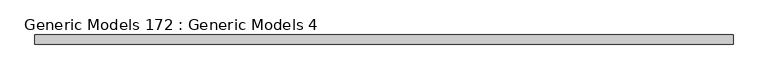
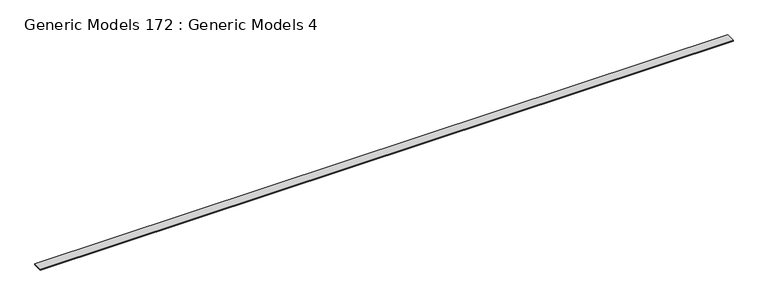
"""IFC4 building model written with IfcOpenShell, lengths in millimetres: proxy geometry, Generic Models 172 : Generic Models 4."""

import ifcopenshell
import ifcopenshell.guid

model = None  # the IFC model being written
_history = None  # IfcOwnerHistory: only IFC2X3 demands one
_inside = {}  # id of a spatial element -> (the spatial element, [elements in it])
_under = {}  # id of a project, library or spatial element -> (it, [spatial elements below it])
_declared = {}  # id of a project -> (the project, [libraries it declares])
_typed = {}  # id of a type object -> (the type object, [elements of that type])
_made_of = {}  # id of a material, layer set ... -> (it, [elements and type objects made of it])


def new_model(schema):
    """Start an empty IFC model of exactly this schema.

    Asked for "IFC4X3", IfcOpenShell would pick the latest addendum, in which some entities
    have other attributes; the version numbers below select the first issue.
    IFC2X3 requires an IfcOwnerHistory on every rooted entity: one is made here for all.
    """
    global model, _history
    if schema == "IFC4X3":
        model = ifcopenshell.file(schema_version=(4, 3, 0, 0))
    else:
        model = ifcopenshell.file(schema=schema)
    _inside.clear()
    _under.clear()
    _declared.clear()
    _typed.clear()
    _made_of.clear()
    _history = None
    if model.schema == "IFC2X3":
        org = make("IfcOrganization", Name="unknown")
        user = make(
            "IfcPersonAndOrganization",
            ThePerson=make("IfcPerson", FamilyName="unknown"),
            TheOrganization=org,
        )
        app = make(
            "IfcApplication",
            ApplicationDeveloper=org,
            Version="unknown",
            ApplicationFullName="unknown",
            ApplicationIdentifier="unknown",
        )
        _history = make(
            "IfcOwnerHistory",
            OwningUser=user,
            OwningApplication=app,
            ChangeAction="ADDED",
            CreationDate=0,
        )
    return model


def make(cls, **values):
    """One entity of the class cls with the attributes given. An attribute that is None is left unset."""
    return model.create_entity(
        cls, **{name: value for name, value in values.items() if value is not None}
    )


def rooted(cls, **values):
    """An entity with a GlobalId (a new one), such as an element, a storey or a relation."""
    return make(cls, GlobalId=ifcopenshell.guid.new(), OwnerHistory=_history, **values)


def si_unit(unit_type, name, prefix=None):
    """IfcSIUnit, for example si_unit("LENGTHUNIT", "METRE", prefix="MILLI")."""
    return make("IfcSIUnit", UnitType=unit_type, Prefix=prefix, Name=name)


def assignment(units):
    """IfcUnitAssignment: the units of a project."""
    return None if units is None else make("IfcUnitAssignment", Units=units)


def point(xyz):
    """IfcCartesianPoint."""
    return None if xyz is None else make("IfcCartesianPoint", Coordinates=xyz)


def direction(xyz):
    """IfcDirection."""
    return None if xyz is None else make("IfcDirection", DirectionRatios=xyz)


def frame(location, z_axis=None, x_axis=None):
    """IfcAxis2Placement3D, a coordinate frame: its origin and axes. An axis left out is left unset."""
    return make(
        "IfcAxis2Placement3D",
        Location=point(location),
        Axis=direction(z_axis),
        RefDirection=direction(x_axis),
    )


def origin():
    """The frame at (0, 0, 0) with its axes left unset."""
    return frame((0.0, 0.0, 0.0))


def place(relative_to, where):
    """IfcLocalPlacement: puts the frame where relative to a parent placement (None: the world)."""
    return make(
        "IfcLocalPlacement", PlacementRelTo=relative_to, RelativePlacement=where
    )


def context(
    kind, dimensions, precision=None, world=None, true_north=None, identifier=None
):
    """IfcGeometricRepresentationContext, for example the 3D "Model" context."""
    return make(
        "IfcGeometricRepresentationContext",
        ContextIdentifier=identifier,
        ContextType=kind,
        CoordinateSpaceDimension=dimensions,
        Precision=precision,
        WorldCoordinateSystem=world,
        TrueNorth=true_north,
    )


def project(units=None, contexts=None):
    """IfcProject with its units and contexts."""
    return rooted(
        "IfcProject",
        Name="project",
        RepresentationContexts=contexts,
        UnitsInContext=assignment(units),
    )


def spatial(cls, under=None, at=None, **own):
    """A site, building, storey or space (cls), placed at a placement, below another one or the project."""
    s = rooted(cls, ObjectPlacement=at, **own)
    if under is not None:
        _under.setdefault(under.id(), (under, []))[1].append(s)
    return s


def polyline(points):
    """IfcPolyline through the points."""
    return make("IfcPolyline", Points=[point(p) for p in points])


def outline(outer, holes=None, kind="AREA"):
    """IfcArbitraryClosedProfileDef: a profile drawn as a closed curve; with holes, ...WithVoids."""
    if holes is None:
        return make("IfcArbitraryClosedProfileDef", ProfileType=kind, OuterCurve=outer)
    return make(
        "IfcArbitraryProfileDefWithVoids",
        ProfileType=kind,
        OuterCurve=outer,
        InnerCurves=holes,
    )


def extrude(swept, where, along, depth):
    """IfcExtrudedAreaSolid: the profile swept, set in the frame where, extruded along a direction by depth."""
    return make(
        "IfcExtrudedAreaSolid",
        SweptArea=swept,
        Position=where,
        ExtrudedDirection=direction(along),
        Depth=depth,
    )


def shape(context_of_items, identifier, shape_type, items):
    """IfcShapeRepresentation: the items that make up one representation, for example the "Body"."""
    return make(
        "IfcShapeRepresentation",
        ContextOfItems=context_of_items,
        RepresentationIdentifier=identifier,
        RepresentationType=shape_type,
        Items=items,
    )


def source(mapping_origin, context_of_items, identifier, shape_type, items):
    """IfcRepresentationMap: a shape defined once, which mapped items show again and again."""
    return make(
        "IfcRepresentationMap",
        MappingOrigin=mapping_origin,
        MappedRepresentation=shape(context_of_items, identifier, shape_type, items),
    )


def transform(
    local_origin,
    x_axis=None,
    y_axis=None,
    z_axis=None,
    scale=None,
    scale2=None,
    scale3=None,
    uniform=True,
):
    """IfcCartesianTransformationOperator3D, or its non-uniform kind. x_axis, y_axis, z_axis: its Axis1, 2, 3."""
    if uniform:
        return make(
            "IfcCartesianTransformationOperator3D",
            Axis1=direction(x_axis),
            Axis2=direction(y_axis),
            LocalOrigin=point(local_origin),
            Scale=scale,
            Axis3=direction(z_axis),
        )
    return make(
        "IfcCartesianTransformationOperator3DnonUniform",
        Axis1=direction(x_axis),
        Axis2=direction(y_axis),
        LocalOrigin=point(local_origin),
        Scale=scale,
        Axis3=direction(z_axis),
        Scale2=scale2,
        Scale3=scale3,
    )


def mapped(mapping_source, mapping_target):
    """IfcMappedItem: shows the shape of a source again, moved by a transform."""
    return make(
        "IfcMappedItem", MappingSource=mapping_source, MappingTarget=mapping_target
    )


def made_of(thing, what):
    """Note that an element or type object is made of a material, layer set ...; save() writes the relation."""
    if what is not None:
        _made_of.setdefault(what.id(), (what, []))[1].append(thing)
    return thing


def element(
    cls,
    number,
    at=None,
    inside=None,
    cuts=None,
    type_object=None,
    material=None,
    context=None,
    identifier="Body",
    shape_type=None,
    held_by="IfcProductDefinitionShape",
    body=None,
    shapes=None,
    **own,
):
    """One element of the class cls, such as IfcWall. Its Tag is "e" and its number.

    at: its placement. inside: the storey or other place that contains it. cuts: it is an
    opening in that element (IfcRelVoidsElement). A single representation is given by context,
    identifier, shape_type and body (its items); several are given by shapes. held_by: the class
    of the entity that holds the representations. save() writes the other relations.
    """
    e = rooted(cls, Tag="e%d" % number, ObjectPlacement=at, **own)
    if body is not None:
        shapes = [shape(context, identifier, shape_type, body)]
    if shapes is not None:
        e.Representation = make(held_by, Representations=shapes)
    if inside is not None:
        _inside.setdefault(inside.id(), (inside, []))[1].append(e)
    if cuts is not None:
        rooted(
            "IfcRelVoidsElement", RelatingBuildingElement=cuts, RelatedOpeningElement=e
        )
    if type_object is not None:
        _typed.setdefault(type_object.id(), (type_object, []))[1].append(e)
    return made_of(e, material)


def aggregate(whole, parts):
    """IfcRelAggregates: a whole, such as a stair, and the parts it consists of."""
    return rooted("IfcRelAggregates", RelatingObject=whole, RelatedObjects=parts)


def save(model, path):
    """Write the relations noted so far, then the file.

    IfcRelAggregates (storeys below a building ...), IfcRelContainedInSpatialStructure (elements
    in a storey), IfcRelDefinesByType, IfcRelAssociatesMaterial and IfcRelDeclares: one each for
    every whole, place, type object, material and project.
    """
    for whole, parts in _under.values():
        aggregate(whole, parts)
    for where, things in _inside.values():
        rooted(
            "IfcRelContainedInSpatialStructure",
            RelatedElements=things,
            RelatingStructure=where,
        )
    for kind, things in _typed.values():
        rooted("IfcRelDefinesByType", RelatedObjects=things, RelatingType=kind)
    for what, things in _made_of.values():
        rooted("IfcRelAssociatesMaterial", RelatedObjects=things, RelatingMaterial=what)
    for by, libraries in _declared.values():
        rooted("IfcRelDeclares", RelatingContext=by, RelatedDefinitions=libraries)
    model.write(path)


def generic_models_172_generic_models_4_ae546b1d(model_context):
    return source(origin(), model_context, "Body", "SweptSolid", [
        extrude(outline(polyline([(2196.9263704, -5471.0980338), (2196.9263704, -5633.3405338), (-10259.9171316, -5633.3405338), (-10259.9171316, -5471.0980338), (2196.9263704, -5471.0980338)])), frame((0.0, 0.0, 126342.327852), z_axis=(0.0, 0.0, 1.0), x_axis=(1.0, 0.0, 0.0)), (0.0, 0.0, 1.0), 17.78),
    ])


if __name__ == "__main__":
    model = new_model("IFC4")
    model_context = context("Model", 3, world=origin())
    ifc_project = project(units=[si_unit("LENGTHUNIT", "METRE", prefix="MILLI")], contexts=[model_context])
    site = spatial("IfcSite", under=ifc_project)
    building = spatial("IfcBuilding", under=site)
    placement = place(None, origin())
    generic_models_172_generic_models_4_shape = generic_models_172_generic_models_4_ae546b1d(model_context)
    element("IfcBuildingElementProxy", 1, Name="Generic Models 172 : Generic Models 4", ObjectType="Generic Models 172 : Generic Models 4", at=placement, inside=building, context=model_context, shape_type="MappedRepresentation", body=[
        mapped(generic_models_172_generic_models_4_shape, transform((0.0, 0.0, 0.0), x_axis=(1.0, 0.0, 0.0), y_axis=(0.0, 1.0, 0.0), z_axis=(0.0, 0.0, 1.0))),
    ])
    save(model, "model.ifc")

# Revit data of these elements
# Element 1 (IfcBuildingElementProxy, "Generic Models 172 : Generic Models 4")
#   Materials on its faces: "_7/8\" SMOOTH TROWEL EXTERIOR STUCCO (COLOR PER OWNER)"
# Materials
#   "_7/8\" SMOOTH TROWEL EXTERIOR STUCCO (COLOR PER OWNER)": class "Generic", colour RGB 233 233 233, transparency 0, Cost = 0
